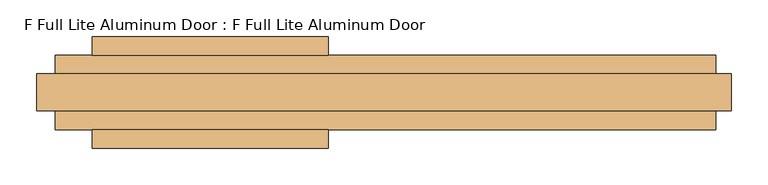
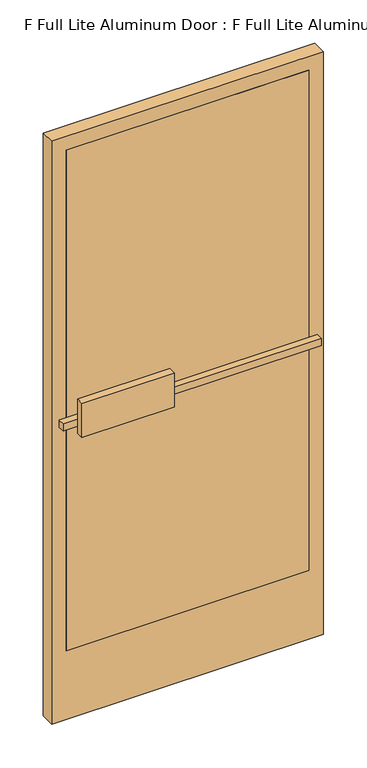
"""IFC4 building model written with IfcOpenShell, lengths in millimetres: door geometry, F Full Lite Aluminum Door : F Full Lite Aluminum Door."""

from ifc_helpers import new_model, si_unit, frame, origin, place, context, project, spatial, polyline, outline, extrude, source, transform, mapped, element, save


def f_full_lite_aluminum_door_f_full_lite_aluminum_door_b58119dc(model_context):
    return source(origin(), model_context, "Body", "SweptSolid", [
        extrude(outline(polyline([(424.259375, 0.0), (424.259375, -50.8), (-424.259375, -50.8), (-424.259375, 0.0), (424.259375, 0.0)])), frame((0.0, 0.0, 254.0), z_axis=(0.0, 0.0, 1.0), x_axis=(1.0, 0.0, 0.0)), (0.0, 0.0, 1.0), 1852.6125),
        extrude(outline(polyline([(2157.4125, -475.059375), (0.0, -475.059375), (0.0, 475.059375), (2157.4125, 475.059375), (2157.4125, -475.059375)]), holes=[polyline([(2106.6125, -424.259375), (2106.6125, 424.259375), (254.0, 424.259375), (254.0, -424.259375), (2106.6125, -424.259375)])]), frame((0.0, -50.8, 0.0), z_axis=(0.0, 1.0, 0.0), x_axis=(0.0, 0.0, 1.0)), (0.0, 0.0, 1.0), 50.8),
        extrude(outline(polyline([(-398.859375, 25.4), (-398.859375, 50.8), (-76.2, 50.8), (-76.2, 25.4), (-398.859375, 25.4)])), frame((0.0, 0.0, 1041.4), z_axis=(0.0, 0.0, 1.0), x_axis=(1.0, 0.0, 0.0)), (0.0, 0.0, 1.0), 127.0),
        extrude(outline(polyline([(-76.2, -76.2), (-76.2, -101.6), (-398.859375, -101.6), (-398.859375, -76.2), (-76.2, -76.2)])), frame((0.0, 0.0, 1065.2125), z_axis=(0.0, 0.0, 1.0), x_axis=(1.0, 0.0, 0.0)), (0.0, 0.0, 1.0), 127.0),
        extrude(outline(polyline([(-449.659375, 0.0), (-449.659375, 25.4), (453.2879464, 25.4), (453.2879464, 0.0), (-449.659375, 0.0)])), frame((0.0, 0.0, 1116.0125), z_axis=(0.0, 0.0, 1.0), x_axis=(1.0, 0.0, 0.0)), (0.0, 0.0, 1.0), 25.4),
        extrude(outline(polyline([(453.2879464, -50.8), (453.2879464, -76.2), (-449.659375, -76.2), (-449.659375, -50.8), (453.2879464, -50.8)])), frame((0.0, 0.0, 1092.2), z_axis=(0.0, 0.0, 1.0), x_axis=(1.0, 0.0, 0.0)), (0.0, 0.0, 1.0), 25.4),
    ])


if __name__ == "__main__":
    model = new_model("IFC4")
    model_context = context("Model", 3, world=origin())
    ifc_project = project(units=[si_unit("LENGTHUNIT", "METRE", prefix="MILLI")], contexts=[model_context])
    site = spatial("IfcSite", under=ifc_project)
    building = spatial("IfcBuilding", under=site)
    placement = place(None, origin())
    f_full_lite_aluminum_door_f_full_lite_aluminum_door_shape = f_full_lite_aluminum_door_f_full_lite_aluminum_door_b58119dc(model_context)
    element("IfcDoor", 1, ObjectType="F Full Lite Aluminum Door : F Full Lite Aluminum Door", at=placement, inside=building, context=model_context, shape_type="MappedRepresentation", body=[
        mapped(f_full_lite_aluminum_door_f_full_lite_aluminum_door_shape, transform((0.0, 0.0, 0.0), x_axis=(1.0, 0.0, 0.0), y_axis=(0.0, 1.0, 0.0), z_axis=(0.0, 0.0, 1.0))),
    ])
    save(model, "model.ifc")

# Revit data of these elements
# Type "F Full Lite Aluminum Door : F Full Lite Aluminum Door"
#   Type Mark = "20"
#   Construction Type Id = "SGL"
#   Assembly Code = "B2030100"
#   Analytic Construction = "Large single-glazed windows"
#   Visual Light Transmittance = 0.9
#   Thermal Resistance (R) = 0.179801 (m²·K)/W
#   Solar Heat Gain Coefficient = 0.86
#   Heat Transfer Coefficient (U) = 5.5617 W/(m²·K)
#   Offset = 0' - 2"
#   Function = 1
#   Handle Material = Aluminum
#   Glazing Material = Glass
# Element 1 (IfcDoor, "F Full Lite Aluminum Door : F Full Lite Aluminum Door")
#   Materials on its faces: "Aluminum", "Glass"
# Materials
#   "Aluminum": class "Metal", colour RGB 247 247 247, transparency 0, Description = "Aluminum 6061", Cost = 0
#   "Glass": class "Unassigned", colour RGB 0 0 255, transparency 0.75
